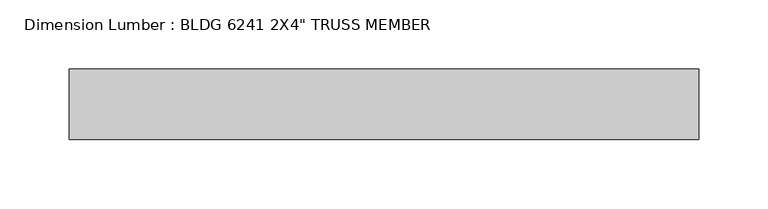
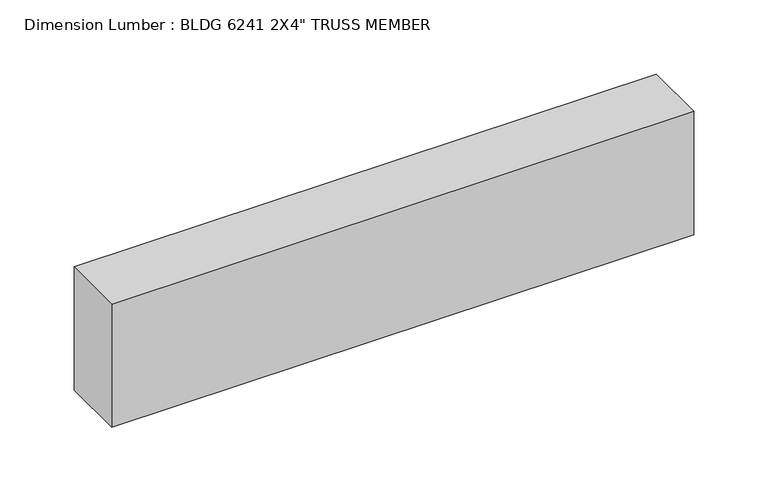
"""IFC4 building model written with IfcOpenShell, lengths in millimetres: beam geometry."""

from ifc_helpers import new_model, si_unit, frame, origin, place, context, project, spatial, polyline, outline, extrude, source, transform, mapped, element, save


def beam_bc99fd75(model_context):
    return source(origin(), model_context, "Body", "SweptSolid", [
        extrude(outline(polyline([(222.3387319, 25.4), (222.3387319, -25.4), (-231.775, -25.4), (-231.775, 25.4), (222.3387319, 25.4)])), frame((0.0, 0.0, -50.8), z_axis=(0.0, 0.0, 1.0), x_axis=(1.0, 0.0, 0.0)), (0.0, 0.0, 1.0), 101.6),
    ])


if __name__ == "__main__":
    model = new_model("IFC4")
    model_context = context("Model", 3, world=origin())
    ifc_project = project(units=[si_unit("LENGTHUNIT", "METRE", prefix="MILLI")], contexts=[model_context])
    site = spatial("IfcSite", under=ifc_project)
    building = spatial("IfcBuilding", under=site)
    placement = place(None, origin())
    beam_shape = beam_bc99fd75(model_context)
    element("IfcBeam", 1, ObjectType="Dimension Lumber : BLDG 6241 2X4\" TRUSS MEMBER", at=placement, inside=building, context=model_context, shape_type="MappedRepresentation", body=[
        mapped(beam_shape, transform((0.0, 0.0, 0.0), x_axis=(1.0, 0.0, 0.0), y_axis=(0.0, 1.0, 0.0), z_axis=(0.0, 0.0, 1.0))),
    ])
    save(model, "model.ifc")

# Revit data of these elements
# Type "Dimension Lumber : BLDG 6241 2X4\" TRUSS MEMBER"
#   Assembly Code = "B10"
#   A = 0.273472 SF
#   Length [instance default] = 5' - 0"
#   b = 0' - 2"
#   d = 0' - 4"
#   Structural Material [instance default] = Softwood, Lumber
# Element 1 (IfcBeam, "Dimension Lumber : BLDG 6241 2X4\" TRUSS MEMBER")
#   Materials on its faces: "Softwood, Lumber"
# Materials
#   "Softwood, Lumber": class "Wood", colour RGB 223 192 134, transparency 0, Description = "Pinus Echinata", Cost = 0
